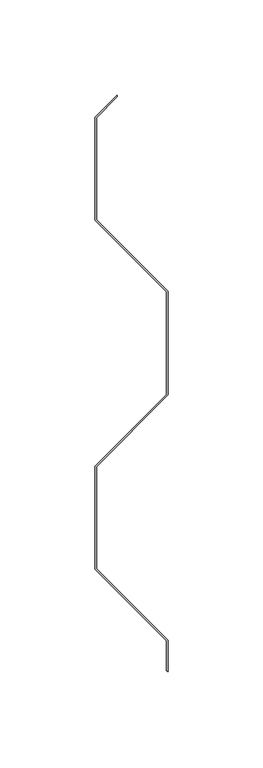
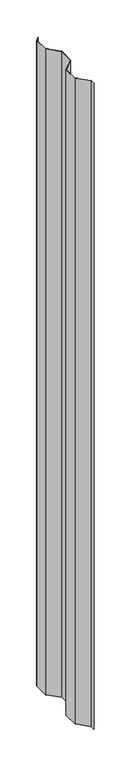
"""IFC4 building model written with IfcOpenShell, lengths in millimetres: proxy geometry, MBCI 7.2-V Panel19 : MBCI 7.2-V Panel-1."""

from ifc_helpers import new_model, si_unit, origin, origin_with_axes, place, context, project, spatial, polyline, outline, extrude, source, transform, mapped, element, save


def generic_models_5c371aaf(model_context):
    return source(origin(), model_context, "Body", "SweptSolid", [
        extrude(outline(polyline([(590353.5827614, -536183.1919067), (590353.5827614, -536129.0801976), (590364.9833956, -536117.6795634), (590365.0253204, -536118.4795376), (590354.1780739, -536129.3267841), (590354.1780739, -536182.9453202), (590391.6684739, -536220.4357202), (590391.6684739, -536274.7163841), (590354.1780739, -536312.2067841), (590354.1780739, -536365.8253202), (590391.6684739, -536403.3157202), (590391.6684739, -536419.8041735), (590391.0731614, -536419.2866763), (590391.0731614, -536403.5623067), (590353.5827614, -536366.0719067), (590353.5827614, -536311.9601976), (590391.0731614, -536274.4697976), (590391.0731614, -536220.6823067), (590353.5827614, -536183.1919067)])), origin_with_axes(), (0.0, 0.0, 1.0), 2438.4),
    ])


if __name__ == "__main__":
    model = new_model("IFC4")
    model_context = context("Model", 3, world=origin())
    ifc_project = project(units=[si_unit("LENGTHUNIT", "METRE", prefix="MILLI")], contexts=[model_context])
    site = spatial("IfcSite", under=ifc_project)
    building = spatial("IfcBuilding", under=site)
    placement = place(None, origin())
    generic_models_shape = generic_models_5c371aaf(model_context)
    element("IfcBuildingElementProxy", 1, Name="MBCI 7.2-V Panel19 : MBCI 7.2-V Panel-1", ObjectType="MBCI 7.2-V Panel19 : MBCI 7.2-V Panel-1", at=placement, inside=building, context=model_context, shape_type="MappedRepresentation", body=[
        mapped(generic_models_shape, transform((0.0, 0.0, 0.0), x_axis=(1.0, 0.0, 0.0), y_axis=(0.0, 1.0, 0.0), z_axis=(0.0, 0.0, 1.0))),
    ])
    save(model, "model.ifc")

# Revit data of these elements
# Element 1 (IfcBuildingElementProxy, "MBCI 7.2-V Panel19 : MBCI 7.2-V Panel-1")
#   Materials on its faces: "MTL PANEL"
# Materials
#   "MTL PANEL": class "Generic", colour RGB 239 242 240, transparency 0, Cost = 0
